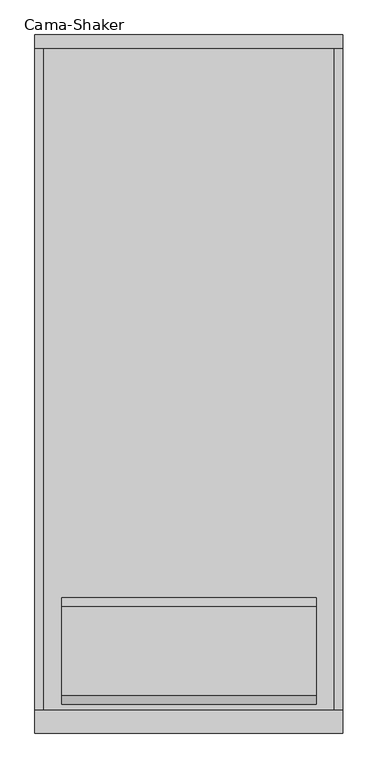
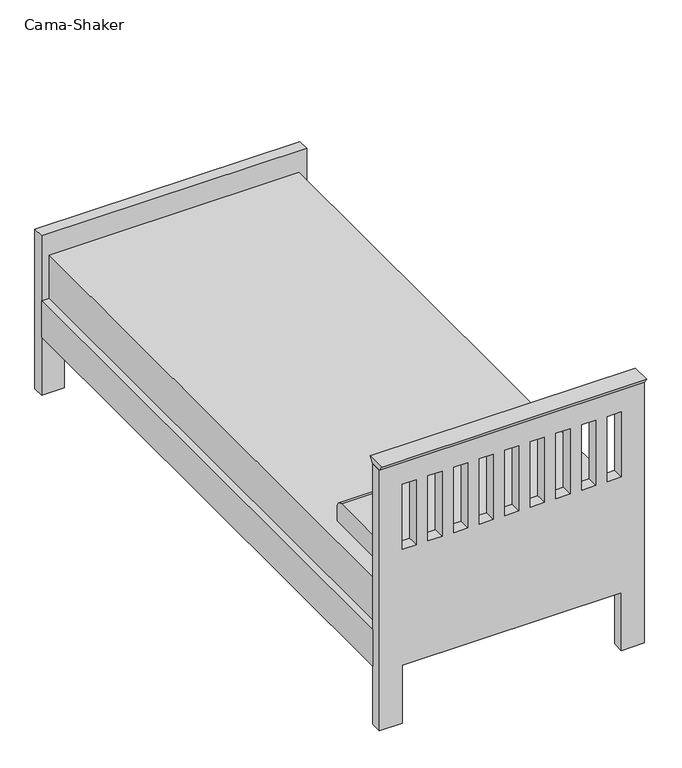
"""IFC4 building model written with IfcOpenShell, lengths in millimetres: furniture geometry, Cama-Shaker : 880 x 1981 mm - Solteiro."""

import ifcopenshell
import ifcopenshell.guid

model = None  # the IFC model being written
_history = None  # IfcOwnerHistory: only IFC2X3 demands one
_inside = {}  # id of a spatial element -> (the spatial element, [elements in it])
_under = {}  # id of a project, library or spatial element -> (it, [spatial elements below it])
_declared = {}  # id of a project -> (the project, [libraries it declares])
_typed = {}  # id of a type object -> (the type object, [elements of that type])
_made_of = {}  # id of a material, layer set ... -> (it, [elements and type objects made of it])


def new_model(schema):
    """Start an empty IFC model of exactly this schema.

    Asked for "IFC4X3", IfcOpenShell would pick the latest addendum, in which some entities
    have other attributes; the version numbers below select the first issue.
    IFC2X3 requires an IfcOwnerHistory on every rooted entity: one is made here for all.
    """
    global model, _history
    if schema == "IFC4X3":
        model = ifcopenshell.file(schema_version=(4, 3, 0, 0))
    else:
        model = ifcopenshell.file(schema=schema)
    _inside.clear()
    _under.clear()
    _declared.clear()
    _typed.clear()
    _made_of.clear()
    _history = None
    if model.schema == "IFC2X3":
        org = make("IfcOrganization", Name="unknown")
        user = make(
            "IfcPersonAndOrganization",
            ThePerson=make("IfcPerson", FamilyName="unknown"),
            TheOrganization=org,
        )
        app = make(
            "IfcApplication",
            ApplicationDeveloper=org,
            Version="unknown",
            ApplicationFullName="unknown",
            ApplicationIdentifier="unknown",
        )
        _history = make(
            "IfcOwnerHistory",
            OwningUser=user,
            OwningApplication=app,
            ChangeAction="ADDED",
            CreationDate=0,
        )
    return model


def make(cls, **values):
    """One entity of the class cls with the attributes given. An attribute that is None is left unset."""
    return model.create_entity(
        cls, **{name: value for name, value in values.items() if value is not None}
    )


def rooted(cls, **values):
    """An entity with a GlobalId (a new one), such as an element, a storey or a relation."""
    return make(cls, GlobalId=ifcopenshell.guid.new(), OwnerHistory=_history, **values)


def si_unit(unit_type, name, prefix=None):
    """IfcSIUnit, for example si_unit("LENGTHUNIT", "METRE", prefix="MILLI")."""
    return make("IfcSIUnit", UnitType=unit_type, Prefix=prefix, Name=name)


def assignment(units):
    """IfcUnitAssignment: the units of a project."""
    return None if units is None else make("IfcUnitAssignment", Units=units)


def point(xyz):
    """IfcCartesianPoint."""
    return None if xyz is None else make("IfcCartesianPoint", Coordinates=xyz)


def direction(xyz):
    """IfcDirection."""
    return None if xyz is None else make("IfcDirection", DirectionRatios=xyz)


def frame(location, z_axis=None, x_axis=None):
    """IfcAxis2Placement3D, a coordinate frame: its origin and axes. An axis left out is left unset."""
    return make(
        "IfcAxis2Placement3D",
        Location=point(location),
        Axis=direction(z_axis),
        RefDirection=direction(x_axis),
    )


def frame_2d(location, x_axis=None):
    """IfcAxis2Placement2D, a coordinate frame in the plane: its origin and x axis."""
    return make(
        "IfcAxis2Placement2D", Location=point(location), RefDirection=direction(x_axis)
    )


def origin():
    """The frame at (0, 0, 0) with its axes left unset."""
    return frame((0.0, 0.0, 0.0))


def place(relative_to, where):
    """IfcLocalPlacement: puts the frame where relative to a parent placement (None: the world)."""
    return make(
        "IfcLocalPlacement", PlacementRelTo=relative_to, RelativePlacement=where
    )


def context(
    kind, dimensions, precision=None, world=None, true_north=None, identifier=None
):
    """IfcGeometricRepresentationContext, for example the 3D "Model" context."""
    return make(
        "IfcGeometricRepresentationContext",
        ContextIdentifier=identifier,
        ContextType=kind,
        CoordinateSpaceDimension=dimensions,
        Precision=precision,
        WorldCoordinateSystem=world,
        TrueNorth=true_north,
    )


def project(units=None, contexts=None):
    """IfcProject with its units and contexts."""
    return rooted(
        "IfcProject",
        Name="project",
        RepresentationContexts=contexts,
        UnitsInContext=assignment(units),
    )


def spatial(cls, under=None, at=None, **own):
    """A site, building, storey or space (cls), placed at a placement, below another one or the project."""
    s = rooted(cls, ObjectPlacement=at, **own)
    if under is not None:
        _under.setdefault(under.id(), (under, []))[1].append(s)
    return s


def polyline(points):
    """IfcPolyline through the points."""
    return make("IfcPolyline", Points=[point(p) for p in points])


def circle_curve(where, radius):
    """IfcCircle in the frame where."""
    return make("IfcCircle", Position=where, Radius=radius)


def trimmed(basis, trim1, trim2, sense, master):
    """IfcTrimmedCurve: the piece of a basis curve between two trims."""
    return make(
        "IfcTrimmedCurve",
        BasisCurve=basis,
        Trim1=trim1,
        Trim2=trim2,
        SenseAgreement=sense,
        MasterRepresentation=master,
    )


def segment(curve, same_sense, transition):
    """IfcCompositeCurveSegment."""
    return make(
        "IfcCompositeCurveSegment",
        Transition=transition,
        SameSense=same_sense,
        ParentCurve=curve,
    )


def composite_curve(segments, self_intersect=None):
    """IfcCompositeCurve: segments joined end to end."""
    return make("IfcCompositeCurve", Segments=segments, SelfIntersect=self_intersect)


def outline(outer, holes=None, kind="AREA"):
    """IfcArbitraryClosedProfileDef: a profile drawn as a closed curve; with holes, ...WithVoids."""
    if holes is None:
        return make("IfcArbitraryClosedProfileDef", ProfileType=kind, OuterCurve=outer)
    return make(
        "IfcArbitraryProfileDefWithVoids",
        ProfileType=kind,
        OuterCurve=outer,
        InnerCurves=holes,
    )


def extrude(swept, where, along, depth):
    """IfcExtrudedAreaSolid: the profile swept, set in the frame where, extruded along a direction by depth."""
    return make(
        "IfcExtrudedAreaSolid",
        SweptArea=swept,
        Position=where,
        ExtrudedDirection=direction(along),
        Depth=depth,
    )


def shape(context_of_items, identifier, shape_type, items):
    """IfcShapeRepresentation: the items that make up one representation, for example the "Body"."""
    return make(
        "IfcShapeRepresentation",
        ContextOfItems=context_of_items,
        RepresentationIdentifier=identifier,
        RepresentationType=shape_type,
        Items=items,
    )


def source(mapping_origin, context_of_items, identifier, shape_type, items):
    """IfcRepresentationMap: a shape defined once, which mapped items show again and again."""
    return make(
        "IfcRepresentationMap",
        MappingOrigin=mapping_origin,
        MappedRepresentation=shape(context_of_items, identifier, shape_type, items),
    )


def transform(
    local_origin,
    x_axis=None,
    y_axis=None,
    z_axis=None,
    scale=None,
    scale2=None,
    scale3=None,
    uniform=True,
):
    """IfcCartesianTransformationOperator3D, or its non-uniform kind. x_axis, y_axis, z_axis: its Axis1, 2, 3."""
    if uniform:
        return make(
            "IfcCartesianTransformationOperator3D",
            Axis1=direction(x_axis),
            Axis2=direction(y_axis),
            LocalOrigin=point(local_origin),
            Scale=scale,
            Axis3=direction(z_axis),
        )
    return make(
        "IfcCartesianTransformationOperator3DnonUniform",
        Axis1=direction(x_axis),
        Axis2=direction(y_axis),
        LocalOrigin=point(local_origin),
        Scale=scale,
        Axis3=direction(z_axis),
        Scale2=scale2,
        Scale3=scale3,
    )


def mapped(mapping_source, mapping_target):
    """IfcMappedItem: shows the shape of a source again, moved by a transform."""
    return make(
        "IfcMappedItem", MappingSource=mapping_source, MappingTarget=mapping_target
    )


def made_of(thing, what):
    """Note that an element or type object is made of a material, layer set ...; save() writes the relation."""
    if what is not None:
        _made_of.setdefault(what.id(), (what, []))[1].append(thing)
    return thing


def element(
    cls,
    number,
    at=None,
    inside=None,
    cuts=None,
    type_object=None,
    material=None,
    context=None,
    identifier="Body",
    shape_type=None,
    held_by="IfcProductDefinitionShape",
    body=None,
    shapes=None,
    **own,
):
    """One element of the class cls, such as IfcWall. Its Tag is "e" and its number.

    at: its placement. inside: the storey or other place that contains it. cuts: it is an
    opening in that element (IfcRelVoidsElement). A single representation is given by context,
    identifier, shape_type and body (its items); several are given by shapes. held_by: the class
    of the entity that holds the representations. save() writes the other relations.
    """
    e = rooted(cls, Tag="e%d" % number, ObjectPlacement=at, **own)
    if body is not None:
        shapes = [shape(context, identifier, shape_type, body)]
    if shapes is not None:
        e.Representation = make(held_by, Representations=shapes)
    if inside is not None:
        _inside.setdefault(inside.id(), (inside, []))[1].append(e)
    if cuts is not None:
        rooted(
            "IfcRelVoidsElement", RelatingBuildingElement=cuts, RelatedOpeningElement=e
        )
    if type_object is not None:
        _typed.setdefault(type_object.id(), (type_object, []))[1].append(e)
    return made_of(e, material)


def aggregate(whole, parts):
    """IfcRelAggregates: a whole, such as a stair, and the parts it consists of."""
    return rooted("IfcRelAggregates", RelatingObject=whole, RelatedObjects=parts)


def save(model, path):
    """Write the relations noted so far, then the file.

    IfcRelAggregates (storeys below a building ...), IfcRelContainedInSpatialStructure (elements
    in a storey), IfcRelDefinesByType, IfcRelAssociatesMaterial and IfcRelDeclares: one each for
    every whole, place, type object, material and project.
    """
    for whole, parts in _under.values():
        aggregate(whole, parts)
    for where, things in _inside.values():
        rooted(
            "IfcRelContainedInSpatialStructure",
            RelatedElements=things,
            RelatingStructure=where,
        )
    for kind, things in _typed.values():
        rooted("IfcRelDefinesByType", RelatedObjects=things, RelatingType=kind)
    for what, things in _made_of.values():
        rooted("IfcRelAssociatesMaterial", RelatedObjects=things, RelatingMaterial=what)
    for by, libraries in _declared.values():
        rooted("IfcRelDeclares", RelatingContext=by, RelatedDefinitions=libraries)
    model.write(path)


def cama_shaker_46b0d072(model_context):
    return source(origin(), model_context, "Body", "SweptSolid", [
        extrude(outline(polyline([(38.1, 914.4), (0.0, 914.4), (-13.8545455, 933.45), (51.9545455, 933.45), (38.1, 914.4)])), frame((-458.8365546, 0.0, 0.0), z_axis=(1.0, 0.0, 0.0), x_axis=(0.0, 1.0, 0.0)), (0.0, 0.0, 1.0), 880.0533613),
        extrude(outline(composite_curve([segment(polyline([(373.2486637, 482.6), (68.4486637, 482.6), (68.4486637, 533.4)]), True, "CONTINUOUS"), segment(trimmed(circle_curve(frame_2d((93.8486637, 533.4)), 25.4), [point((68.4486637, 533.4))], [point((93.8486637, 558.8))], False, "CARTESIAN"), True, "CONTINUOUS"), segment(polyline([(93.8486637, 558.8), (347.8486637, 558.8)]), True, "CONTINUOUS"), segment(trimmed(circle_curve(frame_2d((347.8486637, 533.4)), 25.4), [point((347.8486637, 558.8))], [point((373.2486637, 533.4))], False, "CARTESIAN"), True, "CONTINUOUS"), segment(polyline([(373.2486637, 533.4), (373.2486637, 482.6)]), True, "CONTINUOUS")], self_intersect=False)), frame((-382.85, 0.0, 0.0), z_axis=(1.0, 0.0, 0.0), x_axis=(0.0, 1.0, 0.0)), (0.0, 0.0, 1.0), 727.6),
        extrude(outline(polyline([(395.55, 38.1), (-433.65, 38.1), (-433.65, 1943.1), (395.55, 1943.1), (395.55, 38.1)])), frame((0.0, 0.0, 228.6), z_axis=(0.0, 0.0, 1.0), x_axis=(1.0, 0.0, 0.0)), (0.0, 0.0, 1.0), 254.0),
        extrude(outline(polyline([(395.55, 1943.1), (420.95, 1943.1), (420.95, 38.1), (395.55, 38.1), (395.55, 1943.1)])), frame((0.0, 0.0, 203.0994861), z_axis=(0.0, 0.0, 1.0), x_axis=(1.0, 0.0, 0.0)), (0.0, 0.0, 1.0), 127.0),
        extrude(outline(polyline([(-459.05, 1943.1), (-433.65, 1943.1), (-433.65, 38.1), (-459.05, 38.1), (-459.05, 1943.1)])), frame((0.0, 0.0, 203.5755296), z_axis=(0.0, 0.0, 1.0), x_axis=(1.0, 0.0, 0.0)), (0.0, 0.0, 1.0), 127.0),
        extrude(outline(polyline([(0.0, -382.85), (203.2, -382.85), (203.2, 344.75), (0.0, 344.75), (0.0, 420.95), (558.8, 420.95), (558.8, -459.05), (0.0, -459.05), (0.0, -382.85)])), frame((0.0, 1943.1, 0.0), z_axis=(0.0, 1.0, 0.0), x_axis=(0.0, 0.0, 1.0)), (0.0, 0.0, 1.0), 38.1),
        extrude(outline(polyline([(914.4, 421.2168067), (914.4, -458.8365546), (0.0, -458.8365546), (0.0, -382.85), (203.2, -382.85), (203.2, 344.75), (0.0, 344.75), (0.0, 421.2168067), (914.4, 421.2168067)]), holes=[polyline([(838.2, -335.8722222), (609.6, -335.8722222), (609.6, -382.85), (838.2, -382.85), (838.2, -335.8722222)]), polyline([(838.2, -250.7944444), (609.6, -250.7944444), (609.6, -297.7722222), (838.2, -297.7722222), (838.2, -250.7944444)]), polyline([(838.2, -165.7166667), (609.6, -165.7166667), (609.6, -212.6944444), (838.2, -212.6944444), (838.2, -165.7166667)]), polyline([(838.2, -80.6388889), (609.6, -80.6388889), (609.6, -127.6166667), (838.2, -127.6166667), (838.2, -80.6388889)]), polyline([(838.2, 89.5166667), (609.6, 89.5166667), (609.6, 42.5388889), (838.2, 42.5388889), (838.2, 89.5166667)]), polyline([(838.2, 174.5944444), (609.6, 174.5944444), (609.6, 127.6166667), (838.2, 127.6166667), (838.2, 174.5944444)]), polyline([(838.2, 259.6722222), (609.6, 259.6722222), (609.6, 212.6944444), (838.2, 212.6944444), (838.2, 259.6722222)]), polyline([(838.2, 344.75), (609.6, 344.75), (609.6, 297.7722222), (838.2, 297.7722222), (838.2, 344.75)]), polyline([(838.2, 4.4388889), (609.6, 4.4388889), (609.6, -42.5388889), (838.2, -42.5388889), (838.2, 4.4388889)])]), frame((0.0, 0.0, 0.0), z_axis=(0.0, 1.0, 0.0), x_axis=(0.0, 0.0, 1.0)), (0.0, 0.0, 1.0), 38.1),
    ])


if __name__ == "__main__":
    model = new_model("IFC4")
    model_context = context("Model", 3, world=origin())
    ifc_project = project(units=[si_unit("LENGTHUNIT", "METRE", prefix="MILLI")], contexts=[model_context])
    site = spatial("IfcSite", under=ifc_project)
    building = spatial("IfcBuilding", under=site)
    placement = place(None, origin())
    cama_shaker_shape = cama_shaker_46b0d072(model_context)
    element("IfcFurniture", 1, ObjectType="Cama-Shaker : 880 x 1981 mm - Solteiro", at=placement, inside=building, context=model_context, shape_type="MappedRepresentation", body=[
        mapped(cama_shaker_shape, transform((0.0, 0.0, 0.0), x_axis=(1.0, 0.0, 0.0), y_axis=(0.0, 1.0, 0.0), z_axis=(0.0, 0.0, 1.0))),
    ])
    save(model, "model.ifc")

# Revit data of these elements
# Type "Cama-Shaker : 880 x 1981 mm - Solteiro"
#   Comprimento = 1.9812 m
#   Largura = 0.88 m
#   Material da moldura = wood brown
#   Material do colchão = Linho, branco
#   Default Elevation = 0
# Element 1 (IfcFurniture, "Cama-Shaker : 880 x 1981 mm - Solteiro")
#   Materials on its faces: "wood brown", "Linho, branco"
# Materials
#   "wood brown": class "Wood", colour RGB 80 39 12, transparency 0, Cost = 0
#   "Linho, branco": class "Tecido", colour RGB 247 247 239, transparency 0, Description = "Linho, branco", Cost = 0
